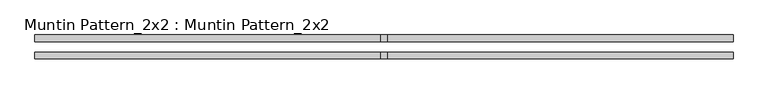
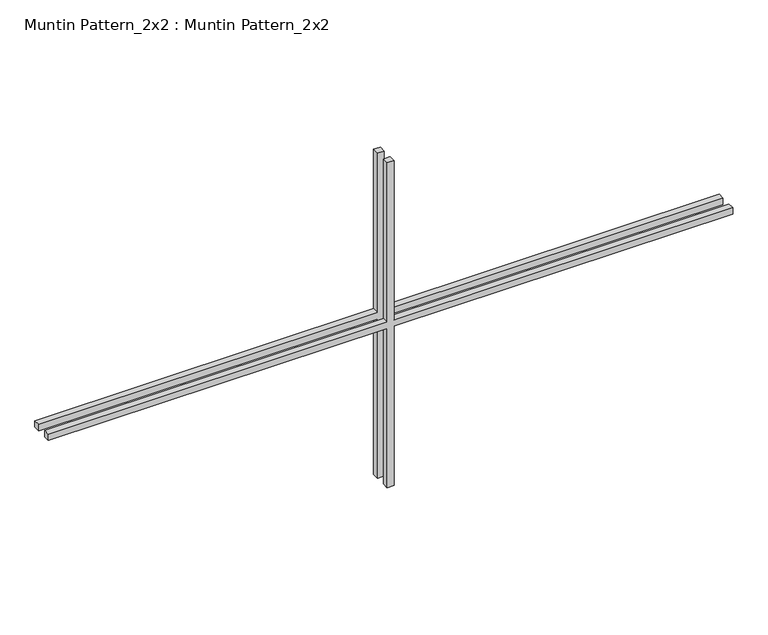
"""IFC4 building model written with IfcOpenShell, lengths in millimetres: proxy geometry, Muntin Pattern_2x2 : Muntin Pattern_2x2."""

from ifc_helpers import new_model, si_unit, frame, origin, place, context, project, spatial, polyline, outline, extrude, source, transform, mapped, element, save


def muntin_pattern_2x2_muntin_pattern_2x2_56bcf098(model_context):
    return source(origin(), model_context, "Body", "SweptSolid", [
        extrude(outline(polyline([(331.7875, -6.35), (331.7875, -647.7), (319.0875, -647.7), (319.0875, -6.35), (0.0, -6.35), (0.0, 6.35), (319.0875, 6.35), (319.0875, 647.7), (331.7875, 647.7), (331.7875, 6.35), (650.875, 6.35), (650.875, -6.35), (331.7875, -6.35)])), frame((0.0, 9.525, 0.0), z_axis=(0.0, 1.0, 0.0), x_axis=(0.0, 0.0, 1.0)), (0.0, 0.0, 1.0), 12.7),
        extrude(outline(polyline([(331.7875, -6.35), (331.7875, -647.7), (319.0875, -647.7), (319.0875, -6.35), (0.0, -6.35), (0.0, 6.35), (319.0875, 6.35), (319.0875, 647.7), (331.7875, 647.7), (331.7875, 6.35), (650.875, 6.35), (650.875, -6.35), (331.7875, -6.35)])), frame((0.0, -22.225, 0.0), z_axis=(0.0, 1.0, 0.0), x_axis=(0.0, 0.0, 1.0)), (0.0, 0.0, 1.0), 12.7),
    ])


if __name__ == "__main__":
    model = new_model("IFC4")
    model_context = context("Model", 3, world=origin())
    ifc_project = project(units=[si_unit("LENGTHUNIT", "METRE", prefix="MILLI")], contexts=[model_context])
    site = spatial("IfcSite", under=ifc_project)
    building = spatial("IfcBuilding", under=site)
    placement = place(None, origin())
    muntin_pattern_2x2_muntin_pattern_2x2_shape = muntin_pattern_2x2_muntin_pattern_2x2_56bcf098(model_context)
    element("IfcBuildingElementProxy", 1, Name="Muntin Pattern_2x2 : Muntin Pattern_2x2", ObjectType="Muntin Pattern_2x2 : Muntin Pattern_2x2", at=placement, inside=building, context=model_context, shape_type="MappedRepresentation", body=[
        mapped(muntin_pattern_2x2_muntin_pattern_2x2_shape, transform((0.0, 0.0, 0.0), x_axis=(1.0, 0.0, 0.0), y_axis=(0.0, 1.0, 0.0), z_axis=(0.0, 0.0, 1.0))),
    ])
    save(model, "model.ifc")

# Revit data of these elements
# Type "Muntin Pattern_2x2 : Muntin Pattern_2x2"
#   Width [instance default] = 4' - 0"
#   Thickness = 0' - 0 1/2"
#   Height [instance default] = 4' - 0"
#   Distance = 0' - 0 3/4"
#   Interior Material [instance default] = none
#   Exterior Material [instance default] = none
# Element 1 (IfcBuildingElementProxy, "Muntin Pattern_2x2 : Muntin Pattern_2x2")
#   Width = 4' - 3"
#   Height = 2' - 1 5/8"
#   Interior Material = Wood - Stained
#   Exterior Material = Clad - White
#   Materials on its faces: "Clad - White", "Wood - Stained"
# Materials
#   "Clad - White": class "Wood", colour RGB 242 242 238, transparency 0, Cost = 0
#   "Wood - Stained": class "Wood", colour RGB 224 178 126, transparency 0, Cost = 0
